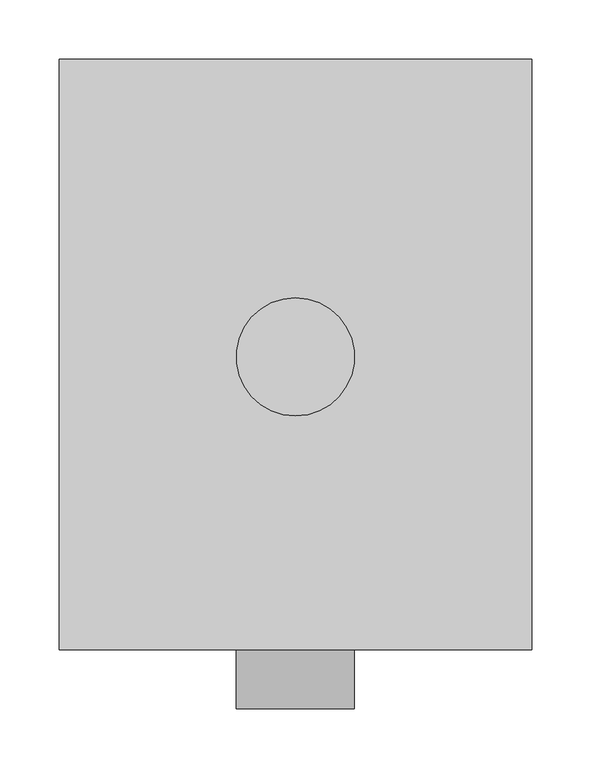
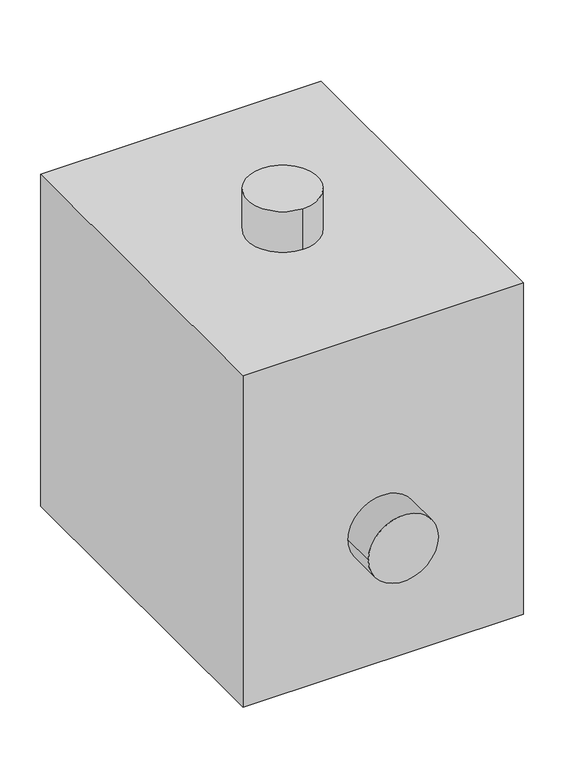
"""IFC4 building model written with IfcOpenShell, lengths in millimetres: proxy geometry, SAN-ARQUETA_BOMBEO : SAN-ARQUETA_BOMBEO."""

from ifc_helpers import new_model, si_unit, point, frame, frame_2d, origin, origin_with_axes, place, context, project, spatial, polyline, circle_curve, trimmed, segment, composite_curve, outline, extrude, source, transform, mapped, element, save


def mechanical_equipment_22a0b1b1(model_context):
    return source(origin(), model_context, "Body", "SweptSolid", [
        extrude(outline(composite_curve([segment(trimmed(circle_curve(frame_2d((0.0, -2.0915789)), 50.0), [point((0.0, -52.0915789))], [point((0.0, 47.9084211))], False, "CARTESIAN"), True, "CONTINUOUS"), segment(trimmed(circle_curve(frame_2d((0.0, -2.0915789)), 50.0), [point((0.0, 47.9084211))], [point((0.0, -52.0915789))], False, "CARTESIAN"), True, "CONTINUOUS")], self_intersect=False)), origin_with_axes(), (0.0, 0.0, 1.0), 61.7447695),
        extrude(outline(composite_curve([segment(trimmed(circle_curve(frame_2d((-300.0, 0.0)), 50.0), [point((-300.0, 50.0))], [point((-300.0, -50.0))], False, "CARTESIAN"), True, "CONTINUOUS"), segment(trimmed(circle_curve(frame_2d((-300.0, 0.0)), 50.0), [point((-300.0, -50.0))], [point((-300.0, 50.0))], False, "CARTESIAN"), True, "CONTINUOUS")], self_intersect=False)), frame((0.0, -300.0, 0.0), z_axis=(0.0, 1.0, 0.0), x_axis=(0.0, 0.0, 1.0)), (0.0, 0.0, 1.0), 50.0),
        extrude(outline(polyline([(200.0, 250.0), (200.0, -250.0), (-200.0, -250.0), (-200.0, 250.0), (200.0, 250.0)])), frame((0.0, 0.0, -500.0), z_axis=(0.0, 0.0, 1.0), x_axis=(1.0, 0.0, 0.0)), (0.0, 0.0, 1.0), 500.0),
    ])


if __name__ == "__main__":
    model = new_model("IFC4")
    model_context = context("Model", 3, world=origin())
    ifc_project = project(units=[si_unit("LENGTHUNIT", "METRE", prefix="MILLI")], contexts=[model_context])
    site = spatial("IfcSite", under=ifc_project)
    building = spatial("IfcBuilding", under=site)
    placement = place(None, origin())
    mechanical_equipment_shape = mechanical_equipment_22a0b1b1(model_context)
    element("IfcBuildingElementProxy", 1, Name="SAN-ARQUETA_BOMBEO : SAN-ARQUETA_BOMBEO", ObjectType="SAN-ARQUETA_BOMBEO : SAN-ARQUETA_BOMBEO", at=placement, inside=building, context=model_context, shape_type="MappedRepresentation", body=[
        mapped(mechanical_equipment_shape, transform((0.0, 0.0, 0.0), x_axis=(1.0, 0.0, 0.0), y_axis=(0.0, 1.0, 0.0), z_axis=(0.0, 0.0, 1.0))),
    ])
    save(model, "model.ifc")

# Revit data of these elements
# Type "SAN-ARQUETA_BOMBEO : SAN-ARQUETA_BOMBEO"
#   Uso [instance default] = "Colector"
#   Tabla [instance default] = "ARQUETA"
#   ØS [instance default] = 0.10 m
#   ØE2 [instance default] = 0.10 m
#   ØE1 [instance default] = 0.10 m
#   hS [instance default] = 0.40 m
#   hE1 [instance default] = 0.30 m
#   Profundidad arqueta [instance default] = 0.50 m
#   L (longitud) [instance default] = 0.40 m
#   LR [instance default] = 0.40 m
#   H [instance default] = 0.50 m
#   FB [instance default] = 0.50 m
#   Default Elevation = 1.2192 m
#   A (anchura) [instance default] = 0.50 m
#   Conexión de ventilación = no
#   Conexión de residuos = yes
#   Conexión AF = no
#   Conexión AC = no
#   WFU = 0
# Element 1 (IfcBuildingElementProxy, "SAN-ARQUETA_BOMBEO : SAN-ARQUETA_BOMBEO")
#   hS = 0.931331 m
